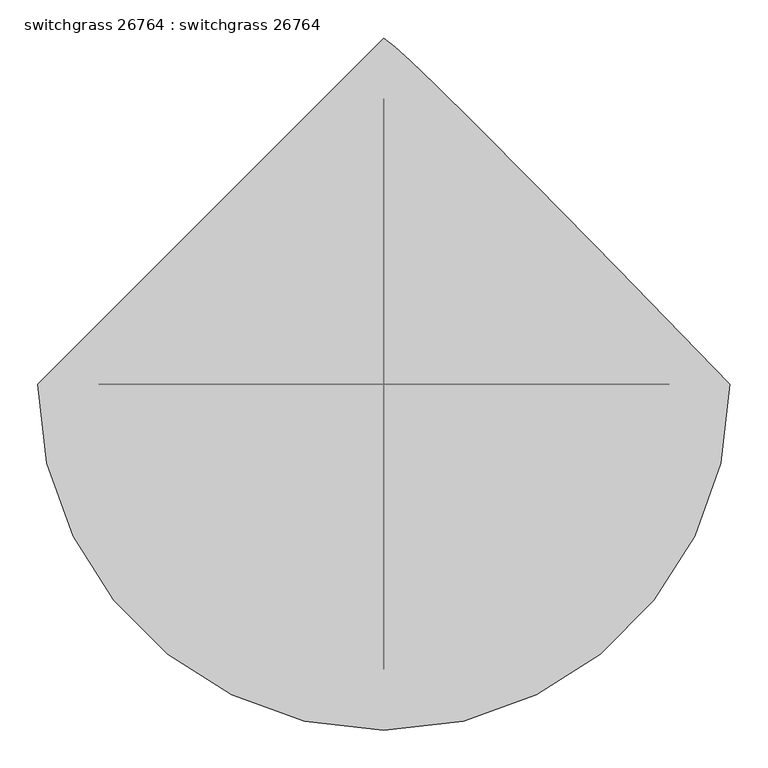
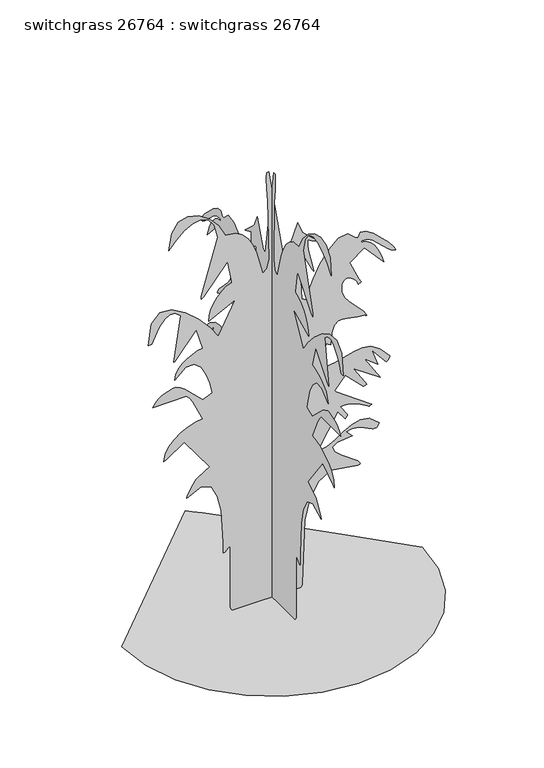
"""IFC4 building model written with IfcOpenShell, lengths in millimetres: proxy geometry, switchgrass 26764 : switchgrass 26764."""

import ifcopenshell
import ifcopenshell.guid

model = None  # the IFC model being written
_history = None  # IfcOwnerHistory: only IFC2X3 demands one
_inside = {}  # id of a spatial element -> (the spatial element, [elements in it])
_under = {}  # id of a project, library or spatial element -> (it, [spatial elements below it])
_declared = {}  # id of a project -> (the project, [libraries it declares])
_typed = {}  # id of a type object -> (the type object, [elements of that type])
_made_of = {}  # id of a material, layer set ... -> (it, [elements and type objects made of it])


def new_model(schema):
    """Start an empty IFC model of exactly this schema.

    Asked for "IFC4X3", IfcOpenShell would pick the latest addendum, in which some entities
    have other attributes; the version numbers below select the first issue.
    IFC2X3 requires an IfcOwnerHistory on every rooted entity: one is made here for all.
    """
    global model, _history
    if schema == "IFC4X3":
        model = ifcopenshell.file(schema_version=(4, 3, 0, 0))
    else:
        model = ifcopenshell.file(schema=schema)
    _inside.clear()
    _under.clear()
    _declared.clear()
    _typed.clear()
    _made_of.clear()
    _history = None
    if model.schema == "IFC2X3":
        org = make("IfcOrganization", Name="unknown")
        user = make(
            "IfcPersonAndOrganization",
            ThePerson=make("IfcPerson", FamilyName="unknown"),
            TheOrganization=org,
        )
        app = make(
            "IfcApplication",
            ApplicationDeveloper=org,
            Version="unknown",
            ApplicationFullName="unknown",
            ApplicationIdentifier="unknown",
        )
        _history = make(
            "IfcOwnerHistory",
            OwningUser=user,
            OwningApplication=app,
            ChangeAction="ADDED",
            CreationDate=0,
        )
    return model


def make(cls, **values):
    """One entity of the class cls with the attributes given. An attribute that is None is left unset."""
    return model.create_entity(
        cls, **{name: value for name, value in values.items() if value is not None}
    )


def rooted(cls, **values):
    """An entity with a GlobalId (a new one), such as an element, a storey or a relation."""
    return make(cls, GlobalId=ifcopenshell.guid.new(), OwnerHistory=_history, **values)


def si_unit(unit_type, name, prefix=None):
    """IfcSIUnit, for example si_unit("LENGTHUNIT", "METRE", prefix="MILLI")."""
    return make("IfcSIUnit", UnitType=unit_type, Prefix=prefix, Name=name)


def assignment(units):
    """IfcUnitAssignment: the units of a project."""
    return None if units is None else make("IfcUnitAssignment", Units=units)


def point(xyz):
    """IfcCartesianPoint."""
    return None if xyz is None else make("IfcCartesianPoint", Coordinates=xyz)


def direction(xyz):
    """IfcDirection."""
    return None if xyz is None else make("IfcDirection", DirectionRatios=xyz)


def frame(location, z_axis=None, x_axis=None):
    """IfcAxis2Placement3D, a coordinate frame: its origin and axes. An axis left out is left unset."""
    return make(
        "IfcAxis2Placement3D",
        Location=point(location),
        Axis=direction(z_axis),
        RefDirection=direction(x_axis),
    )


def origin():
    """The frame at (0, 0, 0) with its axes left unset."""
    return frame((0.0, 0.0, 0.0))


def place(relative_to, where):
    """IfcLocalPlacement: puts the frame where relative to a parent placement (None: the world)."""
    return make(
        "IfcLocalPlacement", PlacementRelTo=relative_to, RelativePlacement=where
    )


def context(
    kind, dimensions, precision=None, world=None, true_north=None, identifier=None
):
    """IfcGeometricRepresentationContext, for example the 3D "Model" context."""
    return make(
        "IfcGeometricRepresentationContext",
        ContextIdentifier=identifier,
        ContextType=kind,
        CoordinateSpaceDimension=dimensions,
        Precision=precision,
        WorldCoordinateSystem=world,
        TrueNorth=true_north,
    )


def project(units=None, contexts=None):
    """IfcProject with its units and contexts."""
    return rooted(
        "IfcProject",
        Name="project",
        RepresentationContexts=contexts,
        UnitsInContext=assignment(units),
    )


def spatial(cls, under=None, at=None, **own):
    """A site, building, storey or space (cls), placed at a placement, below another one or the project."""
    s = rooted(cls, ObjectPlacement=at, **own)
    if under is not None:
        _under.setdefault(under.id(), (under, []))[1].append(s)
    return s


def point_list(points):
    """IfcCartesianPointList2D or 3D."""
    cls = (
        "IfcCartesianPointList2D" if len(points[0]) == 2 else "IfcCartesianPointList3D"
    )
    return make(cls, CoordList=points)


def triangles(points, corners, closed=None, point_numbers=None):
    """IfcTriangulatedFaceSet: each triangle names its three corners, points numbered from 1."""
    return make(
        "IfcTriangulatedFaceSet",
        Coordinates=point_list(points),
        Closed=closed,
        CoordIndex=corners,
        PnIndex=point_numbers,
    )


def shape(context_of_items, identifier, shape_type, items):
    """IfcShapeRepresentation: the items that make up one representation, for example the "Body"."""
    return make(
        "IfcShapeRepresentation",
        ContextOfItems=context_of_items,
        RepresentationIdentifier=identifier,
        RepresentationType=shape_type,
        Items=items,
    )


def source(mapping_origin, context_of_items, identifier, shape_type, items):
    """IfcRepresentationMap: a shape defined once, which mapped items show again and again."""
    return make(
        "IfcRepresentationMap",
        MappingOrigin=mapping_origin,
        MappedRepresentation=shape(context_of_items, identifier, shape_type, items),
    )


def transform(
    local_origin,
    x_axis=None,
    y_axis=None,
    z_axis=None,
    scale=None,
    scale2=None,
    scale3=None,
    uniform=True,
):
    """IfcCartesianTransformationOperator3D, or its non-uniform kind. x_axis, y_axis, z_axis: its Axis1, 2, 3."""
    if uniform:
        return make(
            "IfcCartesianTransformationOperator3D",
            Axis1=direction(x_axis),
            Axis2=direction(y_axis),
            LocalOrigin=point(local_origin),
            Scale=scale,
            Axis3=direction(z_axis),
        )
    return make(
        "IfcCartesianTransformationOperator3DnonUniform",
        Axis1=direction(x_axis),
        Axis2=direction(y_axis),
        LocalOrigin=point(local_origin),
        Scale=scale,
        Axis3=direction(z_axis),
        Scale2=scale2,
        Scale3=scale3,
    )


def mapped(mapping_source, mapping_target):
    """IfcMappedItem: shows the shape of a source again, moved by a transform."""
    return make(
        "IfcMappedItem", MappingSource=mapping_source, MappingTarget=mapping_target
    )


def made_of(thing, what):
    """Note that an element or type object is made of a material, layer set ...; save() writes the relation."""
    if what is not None:
        _made_of.setdefault(what.id(), (what, []))[1].append(thing)
    return thing


def element(
    cls,
    number,
    at=None,
    inside=None,
    cuts=None,
    type_object=None,
    material=None,
    context=None,
    identifier="Body",
    shape_type=None,
    held_by="IfcProductDefinitionShape",
    body=None,
    shapes=None,
    **own,
):
    """One element of the class cls, such as IfcWall. Its Tag is "e" and its number.

    at: its placement. inside: the storey or other place that contains it. cuts: it is an
    opening in that element (IfcRelVoidsElement). A single representation is given by context,
    identifier, shape_type and body (its items); several are given by shapes. held_by: the class
    of the entity that holds the representations. save() writes the other relations.
    """
    e = rooted(cls, Tag="e%d" % number, ObjectPlacement=at, **own)
    if body is not None:
        shapes = [shape(context, identifier, shape_type, body)]
    if shapes is not None:
        e.Representation = make(held_by, Representations=shapes)
    if inside is not None:
        _inside.setdefault(inside.id(), (inside, []))[1].append(e)
    if cuts is not None:
        rooted(
            "IfcRelVoidsElement", RelatingBuildingElement=cuts, RelatedOpeningElement=e
        )
    if type_object is not None:
        _typed.setdefault(type_object.id(), (type_object, []))[1].append(e)
    return made_of(e, material)


def aggregate(whole, parts):
    """IfcRelAggregates: a whole, such as a stair, and the parts it consists of."""
    return rooted("IfcRelAggregates", RelatingObject=whole, RelatedObjects=parts)


def save(model, path):
    """Write the relations noted so far, then the file.

    IfcRelAggregates (storeys below a building ...), IfcRelContainedInSpatialStructure (elements
    in a storey), IfcRelDefinesByType, IfcRelAssociatesMaterial and IfcRelDeclares: one each for
    every whole, place, type object, material and project.
    """
    for whole, parts in _under.values():
        aggregate(whole, parts)
    for where, things in _inside.values():
        rooted(
            "IfcRelContainedInSpatialStructure",
            RelatedElements=things,
            RelatingStructure=where,
        )
    for kind, things in _typed.values():
        rooted("IfcRelDefinesByType", RelatedObjects=things, RelatingType=kind)
    for what, things in _made_of.values():
        rooted("IfcRelAssociatesMaterial", RelatedObjects=things, RelatingMaterial=what)
    for by, libraries in _declared.values():
        rooted("IfcRelDeclares", RelatingContext=by, RelatedDefinitions=libraries)
    model.write(path)


def switchgrass_26764_switchgrass_26764_1323c538(model_context):
    return source(origin(), model_context, "Body", "Tessellation", [
        triangles([(-457.5348269, 0.0, 5.72e-05), (-445.4393443, -104.8366151, 5.72e-05), (-410.9893759, -201.1121793, 5.72e-05), (-356.9483794, -286.0697479, 5.72e-05), (-286.0697479, -356.9483794, 5.72e-05), (-201.1121793, -410.9893759, 5.72e-05), (-104.8366151, -445.4393443, 5.72e-05), (2e-05, -457.5348269, 5.72e-05), (104.8366151, -445.4393443, 5.72e-05), (201.1124336, -410.9893759, 5.72e-05), (286.0697479, -356.9483794, 5.72e-05), (356.9483794, -286.0697479, 5.72e-05), (410.9893759, -201.1121793, 5.72e-05), (445.4393443, -104.8366151, 5.72e-05), (457.5348269, 4e-05, 5.72e-05), (308.8459013, 152.5179615, 5.72e-05), (198.615602, 264.8099809, 5.72e-05), (120.4339824, 343.5803727, 5.72e-05), (67.8913365, 395.5334879, 5.72e-05), (34.5780016, 427.3748946, 5.72e-05), (14.0840831, 445.8076721, 5.72e-05), (-6e-05, 457.5348269, 5.72e-05), (34.93284, 5.5e-06, 1088.4574717), (36.237382, 5.5e-06, 1088.5946726), (37.9539129, 5.5e-06, 1088.9655075), (39.8896437, 5.5e-06, 1089.5065355), (41.8515379, 5.4e-06, 1090.1567139), (43.6465546, 5.4e-06, 1090.8526743), (45.0816551, 5.3e-06, 1091.5334467), (45.9643001, 5.3e-06, 1092.1353722), (79.0584374, 3e-07, 1176.7097157), (93.7670509, 2.4e-06, 1139.9381956), (141.570056, 5.1e-06, 1095.8133453), (139.9581813, 5e-06, 1096.2705122), (120.3097713, 3.5e-06, 1104.9699812), (109.4510318, 2.7e-06, 1111.5257584), (108.7718309, 3.8e-06, 1094.9344746), (110.1157441, 4.9e-06, 1079.5497305), (124.110375, 9.5e-06, 1020.4566805), (126.8614426, 1.06e-05, 1003.8832008), (124.028585, 1.03e-05, 1007.8913137), (90.0899044, 6.2e-06, 1077.4263136), (82.7355931, 6.2e-06, 1077.4263136), (90.0899044, 1.52e-05, 926.664731), (91.5981517, 1.52e-05, 926.3243448), (93.839948, 1.52e-05, 925.4277426), (96.493992, 1.53e-05, 924.1679358), (99.2384648, 1.54e-05, 922.7353924), (101.7517925, 1.55e-05, 921.3205805), (103.7124104, 1.55e-05, 920.1165842), (104.7985178, 1.56e-05, 919.30893), (110.3578079, 1.41e-05, 944.2085003), (125.3806282, 1.19e-05, 981.1629307), (147.3843723, 9.5e-06, 1022.163553), (173.8869515, 7.3e-06, 1059.1942142), (202.4055415, 5.8e-06, 1084.2512604), (230.4577718, 5.5e-06, 1089.3210817), (255.5618354, 6.8e-06, 1066.3950829), (262.9151293, 6.8e-06, 1066.3950829), (269.3514915, 6.1e-06, 1080.2456909), (285.9199024, 6.4e-06, 1077.2713085), (308.5106383, 7.4e-06, 1062.4834757), (355.3227882, 1.03e-05, 1017.5331671), (371.3222114, 1.13e-05, 997.3934807), (376.9076989, 1.17e-05, 985.4987125), (366.3362148, 1.13e-05, 987.6501074), (353.3212752, 1.07e-05, 997.467168), (306.0061764, 8.2e-06, 1041.5234179), (289.6028898, 7.7e-06, 1050.6166128), (273.9463418, 7.7e-06, 1051.6859516), (270.2709666, 7.9e-06, 1048.0105946), (286.0621357, 8.1e-06, 1044.6704641), (300.011793, 8.7e-06, 1035.6788618), (312.0590046, 9.4e-06, 1022.5750105), (322.1529742, 1.04e-05, 1006.8905754), (330.2352207, 1.14e-05, 990.169721), (336.2473901, 1.23e-05, 973.9468014), (340.1361425, 1.32e-05, 959.7583506), (281.3021792, 9.2e-06, 1025.9481331), (237.175821, 1.12e-05, 992.8519701), (237.8959079, 1.14e-05, 989.6693882), (264.7083701, 1.53e-05, 931.0716568), (271.2971213, 1.6e-05, 919.3597263), (262.201401, 1.58e-05, 915.7986065), (257.5227259, 1.51e-05, 925.7833895), (250.3543407, 1.46e-05, 934.7876364), (241.7117542, 1.42e-05, 941.820928), (232.6099115, 1.39e-05, 945.8899384), (224.0638488, 1.4e-05, 946.014422), (217.0887659, 1.43e-05, 941.1985823), (212.6996442, 1.49e-05, 930.4569414), (212.5952538, 1.63e-05, 907.9474869), (220.1395426, 1.74e-05, 888.4809425), (232.934274, 1.85e-05, 871.1581627), (278.8409195, 2.13e-05, 823.0557209), (288.6554731, 2.24e-05, 805.3188675), (284.9775544, 2.24e-05, 805.3188675), (284.9775544, 2.22e-05, 808.9968407), (261.1244319, 2.2e-05, 811.3030952), (219.0793602, 2.16e-05, 819.2355326), (202.3661725, 2.16e-05, 817.8461552), (189.5122514, 2.22e-05, 808.2093887), (181.2572684, 2.35e-05, 786.8149824), (178.341349, 2.57e-05, 750.1603157), (163.6327264, 2.52e-05, 757.5161167), (156.2784152, 2.96e-05, 683.9730766), (191.325313, 2.94e-05, 687.4935013), (248.5903132, 2.85e-05, 703.0763437), (274.1444584, 2.83e-05, 706.7441431), (299.8746466, 2.85e-05, 702.0628881), (327.443785, 2.96e-05, 684.8417009), (358.5206308, 3.16e-05, 650.8794571), (358.1040865, 3.17e-05, 648.5070728), (356.9788645, 3.19e-05, 645.8020054), (355.3380126, 3.21e-05, 643.0156202), (353.374615, 3.22e-05, 640.4019716), (351.2841903, 3.24e-05, 638.2225988), (349.2598226, 3.24e-05, 636.7265419), (347.4894364, 3.25e-05, 636.1703259), (303.3646043, 2.94e-05, 687.6509771), (321.6983145, 3.25e-05, 637.1100941), (281.4164709, 3.05e-05, 668.6899252), (329.1049481, 3.51e-05, 592.0454756), (248.2070336, 3.18e-05, 647.2014839), (249.7422051, 3.2e-05, 643.9071356), (282.1810136, 3.5e-05, 593.8082314), (288.6554731, 3.55e-05, 584.6896382), (287.7740952, 3.56e-05, 584.486453), (278.9298131, 3.57e-05, 581.2174664), (277.6242605, 3.58e-05, 581.0117014), (222.4671985, 3.25e-05, 636.1703259), (189.3728159, 3.49e-05, 595.7208326), (303.3646043, 3.97e-05, 514.8244623), (302.6254598, 3.97e-05, 514.6872977), (301.5739069, 3.97e-05, 514.3164628), (300.3369185, 3.98e-05, 513.7754348), (299.0364347, 3.98e-05, 513.1252201), (297.7994644, 3.98e-05, 512.4292597), (296.7479115, 3.99e-05, 511.7485236), (296.008767, 3.99e-05, 511.1465618), (285.8436898, 3.91e-05, 517.9918562), (258.9959281, 3.82e-05, 530.9178841), (230.2492453, 3.8e-05, 539.6935839), (217.7123288, 3.81e-05, 541.3522036), (207.7585759, 3.82e-05, 540.564788), (229.8212554, 4.01e-05, 507.4711684), (229.5405858, 4.03e-05, 505.7007823), (228.7854538, 4.04e-05, 503.6738711), (227.6866473, 4.05e-05, 501.5834464), (226.3747361, 4.06e-05, 499.6225923), (224.9802718, 4.07e-05, 497.9817404), (223.6343329, 4.08e-05, 496.8565184), (222.4671985, 4.08e-05, 496.4374306), (200.4042828, 3.9e-05, 525.8556567), (137.8929095, 4.54e-05, 419.2189608), (166.0807783, 4.51e-05, 424.9746051), (192.3560459, 4.44e-05, 438.7921846), (217.6356256, 4.35e-05, 455.4799742), (242.8367037, 4.28e-05, 469.858893), (268.8765023, 4.25e-05, 476.7397593), (296.6716989, 4.29e-05, 470.9409127), (327.1389708, 4.44e-05, 447.2757874), (326.9992627, 4.44e-05, 446.6026817), (318.6350567, 4.45e-05, 435.0634515), (318.0737174, 4.45e-05, 433.928092), (304.8454187, 4.44e-05, 435.7644988), (292.8515469, 4.41e-05, 440.3060094), (269.6842292, 4.35e-05, 451.6369311), (257.0629792, 4.32e-05, 455.5028289), (242.7904856, 4.32e-05, 456.2140137), (226.1443541, 4.34e-05, 452.3125803), (244.5298779, 4.45e-05, 433.928092), (198.3082625, 4.53e-05, 429.3560964), (183.5841612, 4.73e-05, 417.3698367), (191.3966749, 5e-05, 400.5525129), (212.7859943, 5.3e-05, 381.4872886), (260.4513443, 5.75e-05, 346.9661762), (268.8053947, 5.81e-05, 336.6766517), (266.5219404, 5.8e-05, 334.0198371), (261.1066641, 5.8e-05, 333.3340141), (178.1579663, 6e-05, 346.4759809), (140.1265758, 6.16e-05, 322.2393062), (114.9013532, 6.35e-05, 274.7464384), (99.9910624, 6.53e-05, 212.9973368), (92.4787665, 7.02e-05, 12.5836557), (91.8127825, 7.03e-05, 8.321819), (90.5290672, 7.04e-05, 4.9722738), (88.4818266, 7.04e-05, 2.3959441), (85.5242583, 7.04e-05, 0.4537325), (-118.3633693, 7.08e-05, 2.4e-05), (-122.0969169, 7.09e-05, 2.3783469), (-124.6485962, 7.1e-05, 5.1976728), (-126.2274606, 7.11e-05, 8.3395482), (-127.0420366, 7.12e-05, 11.6852833), (-127.3018772, 7.12e-05, 15.1165158), (-126.9912402, 7.13e-05, 21.7608447), (-126.8614426, 5.81e-05, 205.9442608), (-129.3712185, 5.82e-05, 207.0623793), (-132.5175108, 5.83e-05, 205.407811), (-143.2413748, 5.85e-05, 195.0563171), (-146.3985949, 5.86e-05, 193.5589884), (-148.9243673, 5.88e-05, 194.9127939), (-148.7935613, 5.68e-05, 227.8207598), (-154.894379, 5.06e-05, 331.9700349), (-165.8895291, 4.76e-05, 382.8233262), (-185.3575813, 4.54e-05, 419.2723005), (-215.6798221, 4.47e-05, 431.1264825), (-259.2397541, 4.61e-05, 408.1877664), (-259.6156759, 4.59e-05, 410.1283092), (-257.8935608, 4.56e-05, 415.3124405), (-244.622078, 4.41e-05, 440.6336783), (-233.4986654, 4.32e-05, 455.9905171), (-232.2906359, 4.31e-05, 458.4568274), (-228.0976142, 4.28e-05, 462.3633476), (-205.3272926, 4.19e-05, 477.5550802), (-189.3728159, 4.15e-05, 485.4061998), (-266.593048, 3.51e-05, 592.0454756), (-321.7491108, 3.73e-05, 555.2739192), (-329.1049481, 3.75e-05, 551.5960187), (-325.1247405, 3.62e-05, 573.5644452), (-314.238341, 3.5e-05, 593.5542134), (-298.0255225, 3.4e-05, 611.0903887), (-278.058609, 3.31e-05, 625.6979273), (-255.9199894, 3.24e-05, 636.9018219), (-233.1864933, 3.2e-05, 644.2271742), (-211.4357316, 3.18e-05, 647.2014839), (-213.7123368, 3.13e-05, 653.8029705), (-240.9860717, 2.74e-05, 712.3753401), (-250.6378082, 2.7e-05, 726.9625311), (-260.7383544, 2.74e-05, 738.2883659), (-362.9504113, 3.12e-05, 737.0260157), (-353.9791203, 3.02e-05, 749.4745291), (-345.6987391, 2.91e-05, 758.1181149), (-337.7028245, 2.78e-05, 763.9169615), (-329.5900566, 2.65e-05, 767.8437567), (-300.461384, 2.23e-05, 778.026638), (-293.1055467, 2.23e-05, 778.026638), (-278.8536186, 2.33e-05, 770.8663919), (-266.2755528, 2.42e-05, 762.6672558), (-211.4357316, 2.81e-05, 709.7133659), (-182.0185046, 2.74e-05, 720.7445967), (-189.8899537, 2.53e-05, 755.5907982), (-200.3534683, 2.34e-05, 786.4390606), (-215.7232605, 2.17e-05, 814.9480036), (-236.4161108, 2.06e-05, 832.6416183), (-262.8490904, 2.07e-05, 831.0515991), (-295.4347286, 2.24e-05, 801.707024), (-292.5975471, 2.14e-05, 818.2246204), (-284.8327776, 2.06e-05, 832.9972652), (-273.265624, 1.99e-05, 845.8724968), (-259.0162394, 1.93e-05, 856.6852816), (-243.2146603, 1.88e-05, 865.2806145), (-226.9795139, 1.84e-05, 871.5010923), (-211.4357316, 1.82e-05, 875.1840797), (-229.8215097, 1.43e-05, 941.3738623), (-296.0113104, 1.91e-05, 860.4749485), (-299.6866857, 1.91e-05, 860.4749485), (-277.7029984, 1e-05, 1003.3269121), (-294.71337, 9.2e-06, 1017.2435772), (-311.0531794, 9.3e-06, 1017.8481188), (-326.2398251, 9.9e-06, 1008.5745569), (-339.7957927, 1.1e-05, 992.857057), (-351.2410243, 1.22e-05, 974.1270956), (-365.8764682, 1.43e-05, 941.3738623), (-376.9076989, 1.43e-05, 941.3738623), (-367.2226796, 1.04e-05, 1007.1064779), (-341.7211112, 8.7e-06, 1034.375889), (-305.7369704, 8.9e-06, 1031.8511158), (-264.604234, 1.03e-05, 1008.203722), (-223.6538811, 1.25e-05, 972.1078148), (-188.2191436, 1.48e-05, 932.229871), (-163.6329808, 1.69e-05, 897.2464685), (-112.1528291, 1.1e-05, 996.5298706), (-193.0499715, 1.34e-05, 956.0804501), (-191.1398955, 1.24e-05, 973.1822405), (-185.7319771, 1.13e-05, 990.7996971), (-177.3111248, 1.03e-05, 1008.0386158), (-166.3611936, 9.4e-06, 1024.0076265), (-153.3675827, 8.5e-06, 1037.8124525), (-138.8136563, 7.9e-06, 1048.5617237), (-123.1842869, 7.5e-06, 1055.3638521), (-122.7161651, 7.3e-06, 1058.0105656), (-134.2157538, 3.3e-06, 1125.2290644), (-138.2424067, 3.4e-06, 1124.548292), (-207.9053874, 8.4e-06, 1039.524412), (-215.1128872, 8.8e-06, 1033.3014633), (-214.9937629, 6.5e-06, 1043.3674913), (-165.5864953, -2.1e-06, 1216.2397156), (-176.4513299, -4.6e-06, 1258.3223213), (-194.0382833, -6.1e-06, 1282.2669353), (-216.3737477, -6.6e-06, 1290.7911243), (-241.4831526, -6.4e-06, 1286.6001011), (-267.3931445, -5.6e-06, 1272.4143391), (-292.1276449, -4.3e-06, 1250.938615), (-313.7150808, -2.8e-06, 1224.8909317), (-305.8919028, -5.9e-06, 1277.1868675), (-285.2950496, -7.5e-06, 1305.4849949), (-256.2374846, -8e-06, 1313.3996281), (-223.0242321, -7.4e-06, 1304.5427559), (-189.9694546, -6.1e-06, 1282.5285473), (-161.3812832, -4.2e-06, 1250.9716072), (-141.570056, -1.9e-06, 1213.4812357), (-111.003735, -1.7e-06, 1210.2630455), (-90.0827918, -1e-06, 1197.192259), (-72.9868286, 2e-07, 1178.0406664), (-59.2218167, 1.6e-06, 1154.5431181), (-48.2927191, 3.1e-06, 1128.4294504), (-27.578531, 7.7e-06, 1051.6859516), (-15.6259369, 7e-06, 1062.9330849), (-8.9939533, 5.3e-06, 1092.3284563), (-12.8700152, -6.1e-06, 1283.3463753), (-14.1246216, -5.9e-06, 1292.5767712), (-15.1875847, -6.3e-06, 1303.493692), (-16.0281459, -7e-06, 1315.7644547), (-16.6151389, -8.1e-06, 1329.0460567), (-16.9180092, -9.2e-06, 1343.0058151), (-16.9057404, -1.04e-05, 1357.3034889), (-16.5471686, -1.14e-05, 1371.5986919), (-9.1928857, -1.14e-05, 1371.5986919), (-3.16e-05, 34.93284, 1088.4574717), (-3.16e-05, 36.237382, 1088.5946726), (-3.16e-05, 37.9539129, 1088.9655075), (-3.16e-05, 39.8896437, 1089.509079), (-3.16e-05, 41.8515379, 1090.1567139), (-3.16e-05, 43.6465546, 1090.8552177), (-3.16e-05, 45.0819049, 1091.5334467), (-3.16e-05, 45.9643001, 1092.1353722), (-3.16e-05, 79.0586918, 1176.7097157), (-3.16e-05, 93.7673053, 1139.9381956), (-3.16e-05, 141.570056, 1095.8133453), (-3.15e-05, 139.9581813, 1096.2705122), (-3.05e-05, 120.3097713, 1104.9699812), (-3.01e-05, 109.4512861, 1111.5257584), (-3.02e-05, 108.7720852, 1094.9344746), (-3.04e-05, 110.1157441, 1079.5497305), (-3.15e-05, 124.1106294, 1020.4566805), (-3.16e-05, 126.8614426, 1003.8832008), (-3.16e-05, 124.028585, 1007.8913137), (-3.16e-05, 90.0901496, 1077.4263136), (-3.16e-05, 82.7358474, 1077.4263136), (-3.16e-05, 90.0901496, 926.664731), (-3.16e-05, 91.5981517, 926.3243448), (-3.16e-05, 93.8402023, 925.4277426), (-3.16e-05, 96.493992, 924.1679358), (-3.16e-05, 99.2387191, 922.7353924), (-3.16e-05, 101.7517925, 921.3205805), (-3.16e-05, 103.7124104, 920.1165842), (-3.16e-05, 104.7985178, 919.30893), (-3.16e-05, 110.3578079, 944.2085003), (-3.16e-05, 125.3806282, 981.1629307), (-3.16e-05, 147.3846266, 1022.163553), (-3.16e-05, 173.8872059, 1059.1942142), (-3.16e-05, 202.4055415, 1084.2512604), (-3.16e-05, 230.4580261, 1089.3210817), (-3.16e-05, 255.5618354, 1066.3950829), (-3.16e-05, 262.9151293, 1066.3950829), (-3.16e-05, 269.3514915, 1080.2456909), (-3.18e-05, 285.9199024, 1077.2713085), (-3.19e-05, 308.5106383, 1062.4834757), (-3.21e-05, 355.3227882, 1017.5331671), (-3.19e-05, 371.3222114, 997.3934807), (-3.16e-05, 376.9076989, 985.4987125), (-3.14e-05, 366.3362148, 987.6501074), (-3.13e-05, 353.3212752, 997.467168), (-3.14e-05, 306.0061764, 1041.5234179), (-3.15e-05, 289.6028898, 1050.6166128), (-3.16e-05, 273.9463418, 1051.6859516), (-3.16e-05, 270.2709666, 1048.0105946), (-3.16e-05, 286.0621357, 1044.6704641), (-3.16e-05, 300.011793, 1035.6788618), (-3.16e-05, 312.0590046, 1022.5750105), (-3.16e-05, 322.1529742, 1006.8905754), (-3.16e-05, 330.2352207, 990.169721), (-3.16e-05, 336.2473901, 973.9468014), (-3.16e-05, 340.1361425, 959.7583506), (-3.16e-05, 281.3021792, 1025.9481331), (-3.16e-05, 237.175821, 992.8519701), (-3.16e-05, 237.8959079, 989.6693882), (-3.19e-05, 264.7083701, 931.0716568), (-3.19e-05, 271.2971213, 919.3597263), (-3.16e-05, 262.201401, 915.7986065), (-3.15e-05, 257.5227259, 925.7833895), (-3.15e-05, 250.3543407, 934.7876364), (-3.15e-05, 241.7117542, 941.820928), (-3.15e-05, 232.6099115, 945.8924818), (-3.15e-05, 224.0641032, 946.014422), (-3.15e-05, 217.0887659, 941.1985823), (-3.16e-05, 212.6996442, 930.4569414), (-3.16e-05, 212.5955081, 907.9474869), (-3.16e-05, 220.1397969, 888.4809425), (-3.16e-05, 232.934274, 871.1581627), (-3.16e-05, 278.8409195, 823.0557209), (-3.16e-05, 288.6554731, 805.3188675), (-3.16e-05, 284.9775544, 805.3188675), (-3.16e-05, 284.9775544, 808.9968407), (-3.16e-05, 261.1244319, 811.3030952), (-3.16e-05, 219.0796145, 819.2355326), (-3.16e-05, 202.3661725, 817.8461552), (-3.16e-05, 189.5122514, 808.2093887), (-3.16e-05, 181.2575227, 786.8149824), (-3.16e-05, 178.3416033, 750.1603157), (-3.16e-05, 163.6329808, 757.5161167), (-3.16e-05, 156.2786695, 683.9730766), (-3.16e-05, 191.325313, 687.4935013), (-3.16e-05, 248.5905676, 703.0763437), (-3.16e-05, 274.1444584, 706.7441431), (-3.16e-05, 299.8746466, 702.0628881), (-3.16e-05, 327.443785, 684.8417009), (-3.16e-05, 358.5206308, 650.8794571), (-3.16e-05, 358.1040865, 648.5070728), (-3.16e-05, 356.9788645, 645.8020054), (-3.16e-05, 355.3380126, 643.0156202), (-3.16e-05, 353.374615, 640.4019716), (-3.16e-05, 351.2841903, 638.2225988), (-3.16e-05, 349.2598226, 636.7265419), (-3.16e-05, 347.4894364, 636.1703259), (-3.16e-05, 303.3646043, 687.6509771), (-3.17e-05, 321.6983145, 637.1100941), (-3.16e-05, 281.4164709, 668.6899252), (-3.16e-05, 329.1049481, 592.0454756), (-3.16e-05, 248.2072879, 647.2014839), (-3.16e-05, 249.7422051, 643.9071356), (-3.16e-05, 282.1810136, 593.8082314), (-3.16e-05, 288.6554731, 584.6896382), (-3.16e-05, 287.7740952, 584.486453), (-3.16e-05, 278.9298131, 581.2174664), (-3.16e-05, 277.6242605, 581.0117014), (-3.16e-05, 222.4671985, 636.1703259), (-3.16e-05, 189.3728159, 595.7208326), (-3.16e-05, 303.3646043, 514.8244623), (-3.16e-05, 302.6254598, 514.6872977), (-3.16e-05, 301.5739069, 514.3164628), (-3.16e-05, 300.3369185, 513.7754348), (-3.16e-05, 299.0364347, 513.1252201), (-3.16e-05, 297.7994644, 512.4292597), (-3.16e-05, 296.7479115, 511.7485236), (-3.16e-05, 296.0113104, 511.1465618), (-3.12e-05, 285.8436898, 517.9918562), (-3.1e-05, 258.9959281, 530.9178841), (-3.13e-05, 230.2494996, 539.6935839), (-3.15e-05, 217.7125832, 541.3522036), (-3.16e-05, 207.7585759, 540.564788), (-3.16e-05, 229.8215097, 507.4711684), (-3.16e-05, 229.5408401, 505.7007823), (-3.16e-05, 228.7857081, 503.6738711), (-3.16e-05, 227.6866473, 501.5834464), (-3.16e-05, 226.3747361, 499.6225923), (-3.16e-05, 224.9805262, 497.9817404), (-3.16e-05, 223.6343329, 496.8565184), (-3.16e-05, 222.4671985, 496.4374306), (-3.16e-05, 200.4042828, 525.8556567), (-3.16e-05, 137.8929095, 419.2189608), (-3.16e-05, 166.0807783, 424.9771485), (-3.17e-05, 192.3560459, 438.7921846), (-3.18e-05, 217.63588, 455.4799742), (-3.19e-05, 242.8367037, 469.858893), (-3.21e-05, 268.8765023, 476.7397593), (-3.21e-05, 296.6716989, 470.9409127), (-3.22e-05, 327.1389708, 447.2757874), (-3.21e-05, 326.9992627, 446.6026817), (-3.16e-05, 318.6350567, 435.0634515), (-3.16e-05, 318.0737174, 433.928092), (-3.16e-05, 304.8454187, 435.7644988), (-3.16e-05, 292.8540904, 440.3060094), (-3.16e-05, 269.6842292, 451.6369311), (-3.16e-05, 257.0629792, 455.5028289), (-3.16e-05, 242.7904856, 456.2140137), (-3.16e-05, 226.1443541, 452.3125803), (-3.16e-05, 244.5301323, 433.928092), (-3.21e-05, 198.3082625, 429.3560964), (-3.33e-05, 183.5841612, 417.3698367), (-3.51e-05, 191.3969293, 400.5525129), (-3.69e-05, 212.7862487, 381.4872886), (-3.94e-05, 260.4513443, 346.9661762), (-3.94e-05, 268.8053947, 336.6766517), (-3.91e-05, 266.5219404, 334.0198371), (-3.91e-05, 261.1066641, 333.3340141), (-4.18e-05, 178.1579663, 346.4759809), (-4.2e-05, 140.1265758, 322.2393062), (-4.1e-05, 114.9013532, 274.7464384), (-3.92e-05, 99.9910624, 212.9973368), (-3.21e-05, 92.4787665, 12.5836296), (-3.2e-05, 91.8127825, 8.3217934), (-3.19e-05, 90.5293216, 4.9722483), (-3.18e-05, 88.4818266, 2.3959185), (-3.16e-05, 85.5242583, 0.4537071), (-3.19e-05, -118.3631241, 0.0), (-3.22e-05, -122.0966625, 2.378324), (-3.24e-05, -124.6483418, 5.1976479), (-3.27e-05, -126.2272062, 8.3395226), (-3.3e-05, -127.0420366, 11.6852833), (-3.33e-05, -127.3018772, 15.1164896), (-3.38e-05, -126.9912402, 21.7608197), (-3.16e-05, -126.8614426, 205.9442608), (-3.17e-05, -129.3709642, 207.062125), (-3.17e-05, -132.5175108, 205.407811), (-3.13e-05, -143.2413748, 195.0563171), (-3.13e-05, -146.3985949, 193.5589884), (-3.16e-05, -148.924113, 194.9127939), (-3.16e-05, -148.7935613, 227.8207598), (-3.16e-05, -154.8941247, 331.9700349), (-3.16e-05, -165.8895291, 382.8233262), (-3.16e-05, -185.357327, 419.274844), (-3.16e-05, -215.6798221, 431.1264825), (-3.16e-05, -259.2397541, 408.1877664), (-3.16e-05, -259.6156759, 410.1283092), (-3.16e-05, -257.8935608, 415.3124405), (-3.16e-05, -244.6218236, 440.6336783), (-3.16e-05, -233.498411, 455.9905171), (-3.16e-05, -232.2906359, 458.4568274), (-3.16e-05, -228.0976142, 462.3658911), (-3.16e-05, -205.3272926, 477.5550802), (-3.16e-05, -189.3728159, 485.4061998), (-3.16e-05, -266.593048, 592.0454756), (-3.16e-05, -321.7491108, 555.2739192), (-3.16e-05, -329.1049481, 551.5960187), (-3.16e-05, -325.1247405, 573.5644452), (-3.16e-05, -314.238341, 593.5542134), (-3.16e-05, -298.0229791, 611.0903887), (-3.16e-05, -278.058609, 625.6979273), (-3.16e-05, -255.9199894, 636.9018219), (-3.16e-05, -233.186239, 644.2271742), (-3.16e-05, -211.4357316, 647.2014839), (-3.14e-05, -213.7123368, 653.8029705), (-3.1e-05, -240.9858174, 712.3753401), (-3.15e-05, -250.6378082, 726.9625311), (-3.26e-05, -260.7383544, 738.2883659), (-3.63e-05, -362.9504113, 737.0260157), (-3.61e-05, -353.9765768, 749.4745291), (-3.54e-05, -345.6987391, 758.1181149), (-3.45e-05, -337.7028245, 763.9169615), (-3.34e-05, -329.5900566, 767.8437567), (-2.99e-05, -300.461384, 778.026638), (-2.99e-05, -293.1055467, 778.026638), (-3.04e-05, -278.8536186, 770.8663919), (-3.08e-05, -266.2730093, 762.6672558), (-3.16e-05, -211.4357316, 709.7133659), (-3.16e-05, -182.0185046, 720.7445967), (-3.15e-05, -189.8899537, 755.5907982), (-3.15e-05, -200.353214, 786.4390606), (-3.15e-05, -215.7232605, 814.9480036), (-3.14e-05, -236.4161108, 832.6416183), (-3.14e-05, -262.8465652, 831.0515991), (-3.14e-05, -295.4347286, 801.707024), (-3.14e-05, -292.5975471, 818.2246204), (-3.14e-05, -284.8327776, 832.9972652), (-3.15e-05, -273.265624, 845.8724968), (-3.15e-05, -259.0162394, 856.6852816), (-3.15e-05, -243.2146603, 865.2806145), (-3.16e-05, -226.9795139, 871.5010923), (-3.16e-05, -211.4357316, 875.1840797), (-3.16e-05, -229.8212554, 941.3738623), (-3.16e-05, -296.008767, 860.4749485), (-3.16e-05, -299.6866857, 860.4749485), (-3.1e-05, -277.7029984, 1003.3269121), (-3.1e-05, -294.71337, 1017.2435772), (-3.11e-05, -311.0531794, 1017.8481188), (-3.12e-05, -326.2398251, 1008.5745569), (-3.13e-05, -339.7957927, 992.857057), (-3.14e-05, -351.2384809, 974.1270956), (-3.16e-05, -365.8764682, 941.3738623), (-3.16e-05, -376.9076989, 941.3738623), (-3.16e-05, -367.2226796, 1007.1064779), (-3.16e-05, -341.7211112, 1034.375889), (-3.16e-05, -305.7369704, 1031.8511158), (-3.16e-05, -264.604234, 1008.203722), (-3.16e-05, -223.6538811, 972.1078148), (-3.16e-05, -188.2191436, 932.229871), (-3.16e-05, -163.6327264, 897.2464685), (-3.16e-05, -112.1528291, 996.5298706), (-3.16e-05, -193.0499715, 956.0804501), (-3.16e-05, -191.1396412, 973.1822405), (-3.16e-05, -185.7317227, 990.7996971), (-3.16e-05, -177.3108705, 1008.0386158), (-3.16e-05, -166.3611936, 1024.0076265), (-3.16e-05, -153.3673283, 1037.8124525), (-3.16e-05, -138.813402, 1048.5617237), (-3.16e-05, -123.1842869, 1055.3638521), (-3.16e-05, -122.7159107, 1058.0105656), (-3.16e-05, -134.2157538, 1125.2290644), (-3.16e-05, -138.2424067, 1124.548292), (-3.16e-05, -207.9053874, 1039.524412), (-3.16e-05, -215.1128872, 1033.3014633), (-2.99e-05, -214.9935086, 1043.3674913), (-3.16e-05, -165.5864953, 1216.2397156), (-3.16e-05, -176.4510756, 1258.3223213), (-3.15e-05, -194.0382833, 1282.2669353), (-3.15e-05, -216.3737477, 1290.7911243), (-3.15e-05, -241.4828982, 1286.6001011), (-3.14e-05, -267.3931445, 1272.4143391), (-3.14e-05, -292.1276449, 1250.938615), (-3.14e-05, -313.7150808, 1224.8909317), (-3.14e-05, -305.8919028, 1277.1868675), (-3.14e-05, -285.2950496, 1305.4849949), (-3.15e-05, -256.2349411, 1313.3996281), (-3.15e-05, -223.0242321, 1304.5427559), (-3.15e-05, -189.9694546, 1282.5285473), (-3.16e-05, -161.3812832, 1250.9716072), (-3.16e-05, -141.570056, 1213.4812357), (-3.16e-05, -111.003735, 1210.2630455), (-3.16e-05, -90.0825374, 1197.192259), (-3.16e-05, -72.9865742, 1178.0432098), (-3.16e-05, -59.2215669, 1154.5431181), (-3.16e-05, -48.2927191, 1128.4294504), (-3.16e-05, -27.578531, 1051.6859516), (-3.16e-05, -15.6258108, 1062.9330849), (-3.16e-05, -8.9938517, 1092.3284563), (-3.16e-05, -12.869888, 1283.3463753), (-3.23e-05, -14.1245194, 1292.5767712), (-3.26e-05, -15.1874576, 1303.493692), (-3.26e-05, -16.0280449, 1315.7644547), (-3.23e-05, -16.6150378, 1329.0460567), (-3.2e-05, -16.917907, 1343.0058151), (-3.17e-05, -16.9056394, 1357.3034889), (-3.16e-05, -16.5470675, 1371.5986919), (-3.16e-05, -9.1927591, 1371.5986919)], [[21, 22, 1], [20, 21, 1], [19, 20, 1], [18, 19, 1], [17, 18, 1], [17, 1, 2], [17, 2, 3], [17, 3, 4], [16, 17, 4], [16, 4, 5], [16, 5, 6], [16, 6, 7], [16, 7, 8], [16, 8, 9], [16, 9, 10], [16, 10, 11], [16, 11, 12], [15, 16, 12], [14, 15, 12], [13, 14, 12], [122, 123, 124], [39, 40, 41], [77, 78, 79], [76, 77, 79], [32, 33, 34], [32, 34, 35], [32, 35, 36], [75, 76, 79], [294, 295, 296], [120, 121, 122], [74, 75, 79], [246, 247, 248], [246, 248, 249], [73, 74, 79], [30, 31, 32], [132, 133, 134], [285, 286, 287], [171, 172, 173], [246, 249, 250], [218, 219, 220], [64, 65, 66], [230, 231, 232], [230, 232, 233], [230, 233, 234], [230, 234, 235], [132, 134, 135], [230, 235, 236], [230, 236, 237], [230, 237, 238], [230, 238, 239], [273, 274, 275], [273, 275, 276], [273, 276, 277], [132, 135, 136], [72, 73, 79], [132, 136, 137], [273, 277, 278], [132, 137, 138], [217, 218, 220], [217, 220, 221], [217, 221, 222], [217, 222, 223], [126, 127, 128], [103, 104, 105], [229, 230, 239], [229, 239, 240], [132, 138, 139], [207, 208, 209], [207, 209, 210], [207, 210, 211], [273, 278, 279], [30, 32, 36], [30, 36, 37], [228, 229, 240], [293, 294, 296], [293, 296, 297], [293, 297, 298], [292, 293, 298], [292, 298, 299], [291, 292, 299], [291, 299, 300], [290, 291, 300], [289, 290, 300], [289, 300, 301], [288, 289, 301], [288, 301, 302], [132, 139, 140], [132, 140, 141], [132, 141, 142], [132, 142, 143], [132, 143, 144], [132, 144, 145], [64, 66, 67], [63, 64, 67], [256, 257, 258], [255, 256, 258], [273, 279, 280], [264, 265, 266], [263, 264, 266], [262, 263, 266], [262, 266, 267], [261, 262, 267], [261, 267, 268], [260, 261, 268], [259, 260, 268], [259, 268, 269], [258, 259, 269], [255, 258, 269], [255, 269, 270], [255, 270, 271], [254, 255, 271], [254, 271, 272], [82, 83, 84], [82, 84, 85], [273, 280, 281], [71, 72, 79], [63, 67, 68], [62, 63, 68], [62, 68, 69], [61, 62, 69], [61, 69, 70], [60, 61, 70], [59, 60, 70], [207, 211, 212], [96, 97, 98], [95, 96, 98], [95, 98, 99], [317, 318, 319], [317, 319, 23], [316, 317, 23], [315, 316, 23], [314, 315, 23], [313, 314, 23], [312, 313, 23], [311, 312, 23], [310, 311, 23], [246, 250, 251], [245, 246, 251], [245, 251, 252], [82, 85, 86], [82, 86, 87], [81, 82, 87], [30, 37, 38], [95, 99, 100], [39, 41, 42], [38, 39, 42], [30, 38, 42], [30, 42, 43], [81, 87, 88], [94, 95, 100], [309, 310, 23], [227, 228, 240], [217, 223, 224], [59, 70, 71], [245, 252, 253], [177, 178, 179], [177, 179, 180], [177, 180, 181], [176, 177, 181], [175, 176, 181], [71, 79, 80], [284, 285, 287], [284, 287, 288], [284, 288, 302], [284, 302, 303], [283, 284, 303], [283, 303, 304], [283, 304, 305], [283, 305, 306], [283, 306, 307], [282, 283, 307], [282, 307, 308], [281, 282, 308], [273, 281, 308], [152, 153, 154], [151, 152, 154], [150, 151, 154], [149, 150, 154], [148, 149, 154], [147, 148, 154], [146, 147, 154], [145, 146, 154], [164, 165, 166], [94, 100, 101], [58, 59, 71], [58, 71, 80], [118, 119, 120], [117, 118, 120], [116, 117, 120], [115, 116, 120], [114, 115, 120], [113, 114, 120], [112, 113, 120], [111, 112, 120], [110, 111, 120], [93, 94, 101], [109, 110, 120], [109, 120, 122], [108, 109, 122], [108, 122, 124], [107, 108, 124], [126, 128, 129], [126, 129, 130], [125, 126, 130], [125, 130, 131], [124, 125, 131], [107, 124, 131], [107, 131, 132], [106, 107, 132], [30, 43, 44], [29, 30, 44], [28, 29, 44], [27, 28, 44], [26, 27, 44], [25, 26, 44], [24, 25, 44], [23, 24, 44], [309, 23, 44], [308, 309, 44], [273, 308, 44], [272, 273, 44], [161, 162, 163], [161, 163, 164], [161, 164, 166], [161, 166, 167], [160, 161, 167], [160, 167, 168], [160, 168, 169], [159, 160, 169], [159, 169, 170], [158, 159, 170], [158, 170, 171], [158, 171, 173], [157, 158, 173], [156, 157, 173], [156, 173, 174], [81, 88, 89], [244, 245, 253], [244, 253, 254], [201, 202, 203], [200, 201, 203], [199, 200, 203], [198, 199, 203], [207, 212, 213], [207, 213, 214], [206, 207, 214], [206, 214, 215], [206, 215, 216], [57, 58, 80], [56, 57, 80], [55, 56, 80], [54, 55, 80], [53, 54, 80], [53, 80, 81], [53, 81, 89], [53, 89, 90], [52, 53, 90], [52, 90, 91], [51, 52, 91], [51, 91, 92], [51, 92, 93], [51, 93, 101], [51, 101, 102], [244, 254, 272], [243, 244, 272], [243, 272, 44], [242, 243, 44], [241, 242, 44], [217, 224, 225], [216, 217, 225], [216, 225, 226], [51, 102, 103], [51, 103, 105], [241, 44, 45], [241, 45, 46], [241, 46, 47], [241, 47, 48], [241, 48, 49], [241, 49, 50], [241, 50, 51], [241, 51, 105], [241, 105, 106], [241, 106, 132], [241, 132, 145], [241, 145, 154], [241, 154, 155], [240, 241, 155], [227, 240, 155], [226, 227, 155], [216, 226, 155], [206, 216, 155], [205, 206, 155], [204, 205, 155], [203, 204, 155], [198, 203, 155], [197, 198, 155], [175, 181, 182], [174, 175, 182], [156, 174, 182], [155, 156, 182], [197, 155, 182], [197, 182, 183], [197, 183, 184], [196, 197, 184], [196, 184, 185], [196, 185, 186], [196, 186, 187], [196, 187, 188], [196, 188, 189], [196, 189, 190], [195, 196, 190], [194, 195, 190], [194, 190, 191], [194, 191, 192], [194, 192, 193], [419, 420, 421], [336, 337, 338], [374, 375, 376], [373, 374, 376], [329, 330, 331], [329, 331, 332], [329, 332, 333], [372, 373, 376], [591, 592, 593], [417, 418, 419], [371, 372, 376], [543, 544, 545], [543, 545, 546], [370, 371, 376], [327, 328, 329], [429, 430, 431], [582, 583, 584], [468, 469, 470], [543, 546, 547], [515, 516, 517], [361, 362, 363], [527, 528, 529], [527, 529, 530], [527, 530, 531], [527, 531, 532], [429, 431, 432], [527, 532, 533], [527, 533, 534], [527, 534, 535], [527, 535, 536], [570, 571, 572], [570, 572, 573], [570, 573, 574], [429, 432, 433], [369, 370, 376], [429, 433, 434], [570, 574, 575], [429, 434, 435], [514, 515, 517], [514, 517, 518], [514, 518, 519], [514, 519, 520], [423, 424, 425], [400, 401, 402], [526, 527, 536], [526, 536, 537], [429, 435, 436], [504, 505, 506], [504, 506, 507], [504, 507, 508], [570, 575, 576], [327, 329, 333], [327, 333, 334], [525, 526, 537], [590, 591, 593], [590, 593, 594], [590, 594, 595], [589, 590, 595], [589, 595, 596], [588, 589, 596], [588, 596, 597], [587, 588, 597], [586, 587, 597], [586, 597, 598], [585, 586, 598], [585, 598, 599], [429, 436, 437], [429, 437, 438], [429, 438, 439], [429, 439, 440], [429, 440, 441], [429, 441, 442], [361, 363, 364], [360, 361, 364], [553, 554, 555], [552, 553, 555], [570, 576, 577], [561, 562, 563], [560, 561, 563], [559, 560, 563], [559, 563, 564], [558, 559, 564], [558, 564, 565], [557, 558, 565], [556, 557, 565], [556, 565, 566], [555, 556, 566], [552, 555, 566], [552, 566, 567], [552, 567, 568], [551, 552, 568], [551, 568, 569], [379, 380, 381], [379, 381, 382], [570, 577, 578], [368, 369, 376], [360, 364, 365], [359, 360, 365], [359, 365, 366], [358, 359, 366], [358, 366, 367], [357, 358, 367], [356, 357, 367], [504, 508, 509], [393, 394, 395], [392, 393, 395], [392, 395, 396], [614, 615, 616], [614, 616, 320], [613, 614, 320], [612, 613, 320], [611, 612, 320], [610, 611, 320], [609, 610, 320], [608, 609, 320], [607, 608, 320], [543, 547, 548], [542, 543, 548], [542, 548, 549], [379, 382, 383], [379, 383, 384], [378, 379, 384], [327, 334, 335], [392, 396, 397], [336, 338, 339], [335, 336, 339], [327, 335, 339], [327, 339, 340], [378, 384, 385], [391, 392, 397], [606, 607, 320], [524, 525, 537], [514, 520, 521], [356, 367, 368], [542, 549, 550], [474, 475, 476], [474, 476, 477], [474, 477, 478], [473, 474, 478], [472, 473, 478], [368, 376, 377], [581, 582, 584], [581, 584, 585], [581, 585, 599], [581, 599, 600], [580, 581, 600], [580, 600, 601], [580, 601, 602], [580, 602, 603], [580, 603, 604], [579, 580, 604], [579, 604, 605], [578, 579, 605], [570, 578, 605], [449, 450, 451], [448, 449, 451], [447, 448, 451], [446, 447, 451], [445, 446, 451], [444, 445, 451], [443, 444, 451], [442, 443, 451], [461, 462, 463], [391, 397, 398], [355, 356, 368], [355, 368, 377], [415, 416, 417], [414, 415, 417], [413, 414, 417], [412, 413, 417], [411, 412, 417], [410, 411, 417], [409, 410, 417], [408, 409, 417], [407, 408, 417], [390, 391, 398], [406, 407, 417], [406, 417, 419], [405, 406, 419], [405, 419, 421], [404, 405, 421], [423, 425, 426], [423, 426, 427], [422, 423, 427], [422, 427, 428], [421, 422, 428], [404, 421, 428], [404, 428, 429], [403, 404, 429], [327, 340, 341], [326, 327, 341], [325, 326, 341], [324, 325, 341], [323, 324, 341], [322, 323, 341], [321, 322, 341], [320, 321, 341], [606, 320, 341], [605, 606, 341], [570, 605, 341], [569, 570, 341], [458, 459, 460], [458, 460, 461], [458, 461, 463], [458, 463, 464], [457, 458, 464], [457, 464, 465], [457, 465, 466], [456, 457, 466], [456, 466, 467], [455, 456, 467], [455, 467, 468], [455, 468, 470], [454, 455, 470], [453, 454, 470], [453, 470, 471], [378, 385, 386], [541, 542, 550], [541, 550, 551], [498, 499, 500], [497, 498, 500], [496, 497, 500], [495, 496, 500], [504, 509, 510], [504, 510, 511], [503, 504, 511], [503, 511, 512], [503, 512, 513], [354, 355, 377], [353, 354, 377], [352, 353, 377], [351, 352, 377], [350, 351, 377], [350, 377, 378], [350, 378, 386], [350, 386, 387], [349, 350, 387], [349, 387, 388], [348, 349, 388], [348, 388, 389], [348, 389, 390], [348, 390, 398], [348, 398, 399], [541, 551, 569], [540, 541, 569], [540, 569, 341], [539, 540, 341], [538, 539, 341], [514, 521, 522], [513, 514, 522], [513, 522, 523], [348, 399, 400], [348, 400, 402], [538, 341, 342], [538, 342, 343], [538, 343, 344], [538, 344, 345], [538, 345, 346], [538, 346, 347], [538, 347, 348], [538, 348, 402], [538, 402, 403], [538, 403, 429], [538, 429, 442], [538, 442, 451], [538, 451, 452], [537, 538, 452], [524, 537, 452], [523, 524, 452], [513, 523, 452], [503, 513, 452], [502, 503, 452], [501, 502, 452], [500, 501, 452], [495, 500, 452], [494, 495, 452], [472, 478, 479], [471, 472, 479], [453, 471, 479], [452, 453, 479], [494, 452, 479], [494, 479, 480], [494, 480, 481], [493, 494, 481], [493, 481, 482], [493, 482, 483], [493, 483, 484], [493, 484, 485], [493, 485, 486], [493, 486, 487], [492, 493, 487], [491, 492, 487], [491, 487, 488], [491, 488, 489], [491, 489, 490]], closed=False),
    ])


if __name__ == "__main__":
    model = new_model("IFC4")
    model_context = context("Model", 3, world=origin())
    ifc_project = project(units=[si_unit("LENGTHUNIT", "METRE", prefix="MILLI")], contexts=[model_context])
    site = spatial("IfcSite", under=ifc_project)
    building = spatial("IfcBuilding", under=site)
    placement = place(None, origin())
    switchgrass_26764_switchgrass_26764_shape = switchgrass_26764_switchgrass_26764_1323c538(model_context)
    element("IfcBuildingElementProxy", 1, Name="switchgrass 26764 : switchgrass 26764", ObjectType="switchgrass 26764 : switchgrass 26764", at=placement, inside=building, context=model_context, shape_type="MappedRepresentation", body=[
        mapped(switchgrass_26764_switchgrass_26764_shape, transform((0.0, 0.0, 0.0), x_axis=(1.0, 0.0, 0.0), y_axis=(0.0, 1.0, 0.0), z_axis=(0.0, 0.0, 1.0))),
    ])
    save(model, "model.ifc")

# Revit data of these elements
# Type "switchgrass 26764 : switchgrass 26764"
#   built-in parameter 1005195 = "RPC-16-FU2N-0J7X-A2JP-J000-ST1L-LVER-AU"
#   Height = 0
